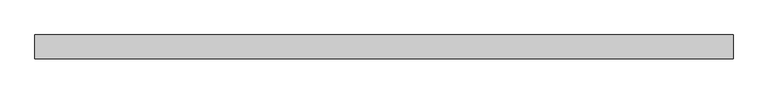
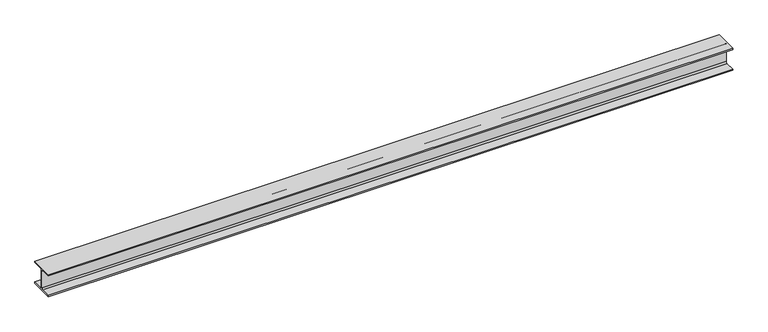
"""IFC4 building model written with IfcOpenShell, lengths in millimetres: beam geometry, 0912_Steel Framing_H-KSD3502 : H_SB_ASB_H-200x200x8x12."""

from ifc_helpers import new_model, si_unit, point, frame, frame_2d, origin, place, context, project, spatial, polyline, circle_curve, trimmed, segment, composite_curve, outline, extrude, source, transform, mapped, element, save


def beam_7b21adab(model_context):
    return source(origin(), model_context, "Body", "SweptSolid", [
        extrude(outline(composite_curve([segment(polyline([(100.0, -88.0), (100.0, -100.0), (-100.0, -100.0), (-100.0, -88.0), (-17.0, -88.0)]), True, "CONTINUOUS"), segment(trimmed(circle_curve(frame_2d((-17.0, -75.0)), 13.0), [point((-17.0, -88.0))], [point((-4.0, -75.0))], True, "CARTESIAN"), True, "CONTINUOUS"), segment(polyline([(-4.0, -75.0), (-4.0, 75.0)]), True, "CONTINUOUS"), segment(trimmed(circle_curve(frame_2d((-17.0, 75.0)), 13.0), [point((-4.0, 75.0))], [point((-17.0, 88.0))], True, "CARTESIAN"), True, "CONTINUOUS"), segment(polyline([(-17.0, 88.0), (-100.0, 88.0), (-100.0, 100.0), (100.0, 100.0), (100.0, 88.0), (17.0, 88.0)]), True, "CONTINUOUS"), segment(trimmed(circle_curve(frame_2d((17.0, 75.0)), 13.0), [point((17.0, 88.0))], [point((4.0, 75.0))], True, "CARTESIAN"), True, "CONTINUOUS"), segment(polyline([(4.0, 75.0), (4.0, -75.0)]), True, "CONTINUOUS"), segment(trimmed(circle_curve(frame_2d((17.0, -75.0)), 13.0), [point((4.0, -75.0))], [point((17.0, -88.0))], True, "CARTESIAN"), True, "CONTINUOUS"), segment(polyline([(17.0, -88.0), (100.0, -88.0)]), True, "CONTINUOUS")], self_intersect=False)), frame((-2907.8125229, 0.0, 0.0), z_axis=(1.0, 0.0, 0.0), x_axis=(0.0, 1.0, 0.0)), (0.0, 0.0, 1.0), 5847.9972501),
    ])


if __name__ == "__main__":
    model = new_model("IFC4")
    model_context = context("Model", 3, world=origin())
    ifc_project = project(units=[si_unit("LENGTHUNIT", "METRE", prefix="MILLI")], contexts=[model_context])
    site = spatial("IfcSite", under=ifc_project)
    building = spatial("IfcBuilding", under=site)
    placement = place(None, origin())
    beam_shape = beam_7b21adab(model_context)
    element("IfcBeam", 1, ObjectType="0912_Steel Framing_H-KSD3502 : H_SB_ASB_H-200x200x8x12", at=placement, inside=building, context=model_context, shape_type="MappedRepresentation", body=[
        mapped(beam_shape, transform((0.0, 0.0, 0.0), x_axis=(1.0, 0.0, 0.0), y_axis=(0.0, 1.0, 0.0), z_axis=(0.0, 0.0, 1.0))),
    ])
    save(model, "model.ifc")

# Revit data of these elements
# Type "0912_Steel Framing_H-KSD3502 : H_SB_ASB_H-200x200x8x12"
#   H_WM Code_1 = "S01AA002-00001 | Main Steel Structure Fabrication Work | Shelter/Building | Medium Steel - Standard (90KG/M>Weight≥30KG/M) | Material: (   )"
#   H_WM Code_2 = "S03AA028-00001 | Main Steel Structure Erection Work | Shelter/Building | Medium Steel (90KG/M>Weight≥30KG/M) | Material: (   )"
#   H_WM Code_3 = "S01AA010-00001 | Main Steel Structure Fabrication Work | Shelter/Building | Steel Painting/Coating | for Non-Fireproofed Steel Surface, Surface Preparation, Primer, Second & Final Coat | Material: (   )"
#   H_Q'ty Cal Type Tag = "SB-Q2"
#   Width = 20.0 cm
#   Web Thickness = 0.8 cm
#   Web Fillet = 1.3 cm
#   Warping Constant = 141000.0 cm⁶
#   W = 0
#   Torsional Moment of Inertia = 26.2485 cm⁴
#   Section Area = 63.53 cm²
#   Plastic Modulus weak axis = 244.0 cm³
#   Plastic Modulus strong axis = 525.0 cm³
#   Perimeter = 1.16 m²/m
#   Nominal Weight = 49.90 kgf/m
#   Moment of Inertia weak axis = 1600.00 cm⁴
#   Moment of Inertia strong axis = 4720.00 cm⁴
#   Height = 20.0 cm
#   Flange Thickness = 1.2 cm
#   Elastic Modulus weak axis = 160.0 cm³
#   Elastic Modulus strong axis = 472.0 cm³
#   Centroid Vertical = 10.0 cm
#   Centroid Horizontal = 10.0 cm
#   Ix = 47200000
#   Length [instance default] = 1.5240 m
#   Zx = 525000
#   b = 0.2000 m
#   h = 0.2000 m
#   r = 0.0130 m
#   s = 0.0080 m
#   t = 0.0120 m
#   A = 0.006353 m²
#   Structural Material [instance default] = Steel, 45-345
#   Assembly Code = ""
# Element 1 (IfcBeam, "0912_Steel Framing_H-KSD3502 : H_SB_ASB_H-200x200x8x12")
#   Structural Material = none
# Materials
#   "Steel, 45-345": class "Metal", colour RGB 189 187 185, transparency 0, Description = "Steel 345 MPa", Cost = 0
